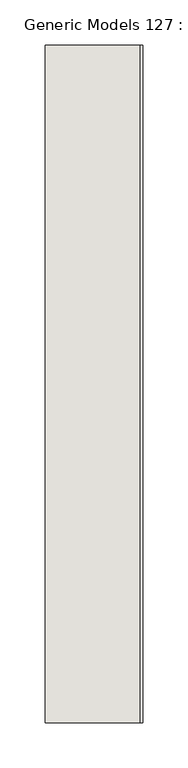
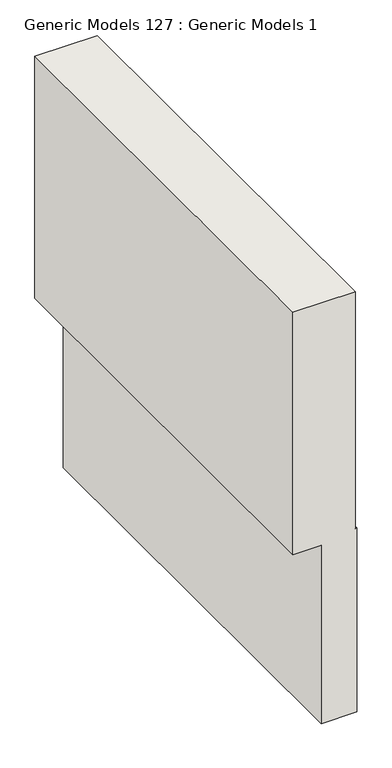
"""IFC4 building model written with IfcOpenShell, lengths in millimetres: wall geometry, Generic Models 127 : Generic Models 1."""

from ifc_helpers import new_model, si_unit, frame, origin, place, context, project, spatial, polyline, outline, extrude, source, transform, mapped, element, save


def generic_models_127_generic_models_1_dc4fc308(model_context):
    return source(origin(), model_context, "Body", "SweptSolid", [
        extrude(outline(polyline([(1866.3462589, 375046.7901825), (1866.3462589, 375107.1151825), (2193.3712588, 375107.1151825), (2193.3712588, 375103.9401825), (2614.4792695, 375103.9401825), (2614.4792695, 374999.1651825), (2183.8462588, 374999.1651825), (2183.8462588, 375046.7901825), (1866.3462589, 375046.7901825)])), frame((0.0, 455.6125, 0.0), z_axis=(0.0, 1.0, 0.0), x_axis=(0.0, 0.0, 1.0)), (0.0, 0.0, 1.0), 750.8875),
    ])


if __name__ == "__main__":
    model = new_model("IFC4")
    model_context = context("Model", 3, world=origin())
    ifc_project = project(units=[si_unit("LENGTHUNIT", "METRE", prefix="MILLI")], contexts=[model_context])
    site = spatial("IfcSite", under=ifc_project)
    building = spatial("IfcBuilding", under=site)
    placement = place(None, origin())
    generic_models_127_generic_models_1_shape = generic_models_127_generic_models_1_dc4fc308(model_context)
    element("IfcWall", 1, ObjectType="Generic Models 127 : Generic Models 1", at=placement, inside=building, context=model_context, shape_type="MappedRepresentation", body=[
        mapped(generic_models_127_generic_models_1_shape, transform((0.0, 0.0, 0.0), x_axis=(1.0, 0.0, 0.0), y_axis=(0.0, 1.0, 0.0), z_axis=(0.0, 0.0, 1.0))),
    ])
    save(model, "model.ifc")

# Revit data of these elements
# Element 1 (IfcWall, "Generic Models 127 : Generic Models 1")
#   Materials on its faces: "SEE SCHEDULE FOR FILLED CORES"
# Materials
#   "SEE SCHEDULE FOR FILLED CORES": class "Generic", colour RGB 170 170 170, transparency 0, Cost = 0
